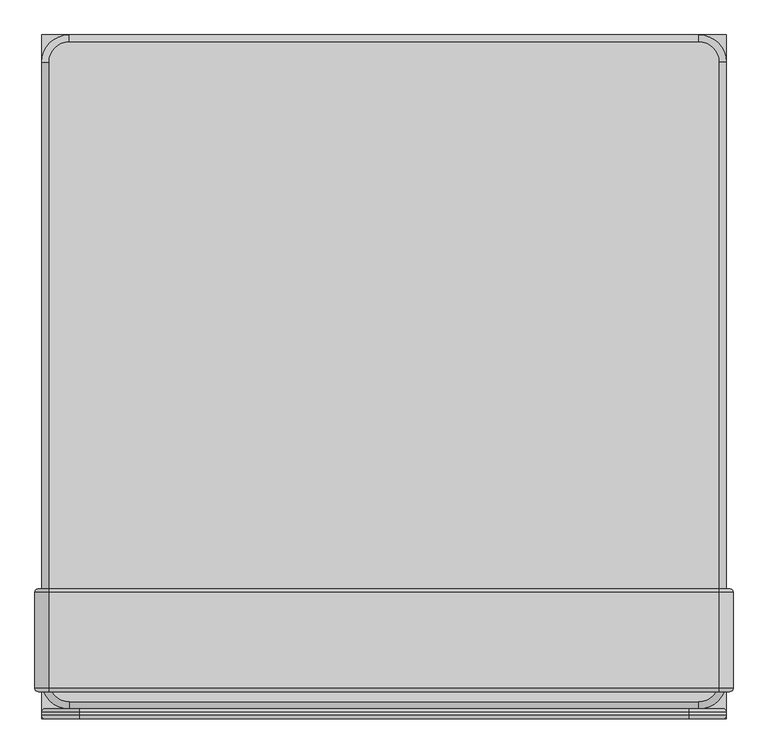
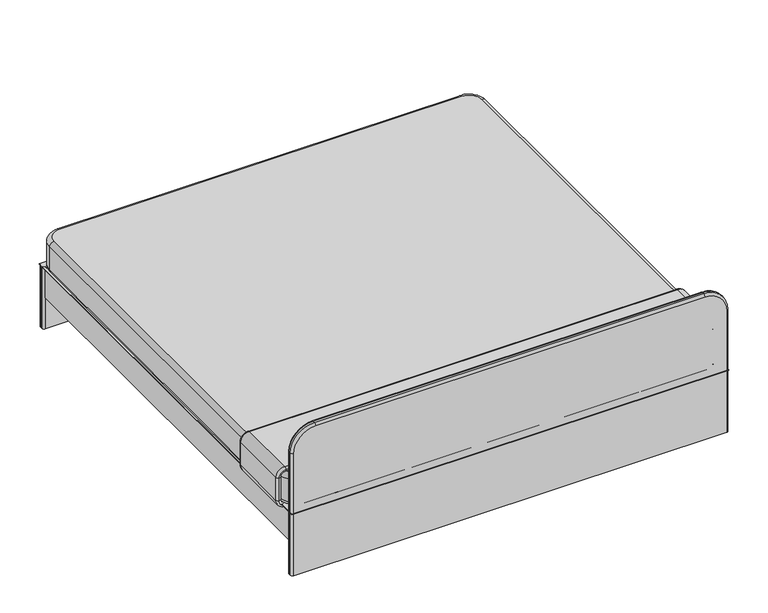
"""IFC4 building model written with IfcOpenShell, lengths in millimetres: furniture geometry, ベッド : 2000 x 2000 mm キング."""

from ifc_helpers import new_model, si_unit, point, frame, frame_2d, origin, origin_with_axes, place, context, project, spatial, polyline, circle_curve, ellipse_curve, trimmed, segment, composite_curve, outline, extrude, source, transform, mapped, element, save
from ifc_brep_helpers import plane_surface, cylinder_surface, revolved_surface, advanced_brep


def furniture_2da6a2a7(model_context):
    return source(origin(), model_context, "Body", "SolidModel", [
        advanced_brep(
        [(1000.0, -960.0, 430.0), (980.0, -960.0, 450.0), (980.0, -680.0, 450.0), (1000.0, -680.0, 430.0), (1010.0, -970.0, 430.0), (980.0, -970.0, 460.0), (1020.0, -960.0, 430.0), (980.0, -960.0, 470.0), (1020.0, -680.0, 430.0), (980.0, -680.0, 470.0), (1010.0, -670.0, 430.0), (980.0, -670.0, 460.0), (1000.0, -680.0, 320.0), (1000.0, -960.0, 320.0), (1010.0, -970.0, 320.0), (1020.0, -960.0, 320.0), (1020.0, -680.0, 320.0), (1010.0, -670.0, 320.0), (980.0, -960.0, 300.0), (980.0, -680.0, 300.0), (980.0, -970.0, 290.0), (980.0, -960.0, 280.0), (980.0, -680.0, 280.0), (980.0, -670.0, 290.0), (-980.0, -680.0, 300.0), (-980.0, -960.0, 300.0), (-980.0, -970.0, 290.0), (-980.0, -960.0, 280.0), (-980.0, -680.0, 280.0), (-980.0, -670.0, 290.0), (-1000.0, -960.0, 320.0), (-1000.0, -680.0, 320.0), (-1010.0, -970.0, 320.0), (-1020.0, -960.0, 320.0), (-1020.0, -680.0, 320.0), (-1010.0, -670.0, 320.0), (-1000.0, -680.0, 430.0), (-1000.0, -960.0, 430.0), (-1010.0, -970.0, 430.0), (-1020.0, -960.0, 430.0), (-1020.0, -680.0, 430.0), (-1010.0, -670.0, 430.0), (-980.0, -960.0, 450.0), (-980.0, -680.0, 450.0), (-980.0, -970.0, 460.0), (-980.0, -960.0, 470.0), (-980.0, -680.0, 470.0), (-980.0, -670.0, 460.0)],
        [
            (0, 1, circle_curve(frame((980.0, -960.0, 430.0), z_axis=(0.0, -1.0, 0.0), x_axis=(0.0, 0.0, 1.0)), 20.0)),
            (1, 2),
            (2, 3, circle_curve(frame((980.0, -680.0, 430.0), z_axis=(0.0, 1.0, 0.0), x_axis=(0.0, 0.0, 1.0)), 20.0)),
            (3, 0),
            (4, 5, circle_curve(frame((980.0, -970.0, 430.0), z_axis=(0.0, -1.0, 0.0), x_axis=(0.0, 0.0, 1.0)), 30.0)),
            (5, 1, circle_curve(frame((980.0, -960.0, 460.0), z_axis=(1.0, 0.0, 0.0), x_axis=(0.0, 0.0, 1.0)), 10.0)),
            (0, 4, circle_curve(frame((1010.0, -960.0, 430.0), z_axis=(0.0, 0.0, 1.0), x_axis=(1.0, 0.0, 0.0)), 10.0)),
            (6, 7, circle_curve(frame((980.0, -960.0, 430.0), z_axis=(0.0, -1.0, 0.0), x_axis=(0.0, 0.0, 1.0)), 40.0)),
            (7, 5, circle_curve(frame((980.0, -960.0, 460.0), z_axis=(1.0, 0.0, 0.0), x_axis=(0.0, 0.0, 1.0)), 10.0)),
            (4, 6, circle_curve(frame((1010.0, -960.0, 430.0), z_axis=(0.0, 0.0, 1.0), x_axis=(1.0, 0.0, 0.0)), 10.0)),
            (8, 9, circle_curve(frame((980.0, -680.0, 430.0), z_axis=(0.0, -1.0, 0.0), x_axis=(0.0, 0.0, 1.0)), 40.0)),
            (9, 7),
            (6, 8),
            (10, 11, circle_curve(frame((980.0, -670.0, 430.0), z_axis=(0.0, -1.0, 0.0), x_axis=(0.0, 0.0, 1.0)), 30.0)),
            (11, 9, circle_curve(frame((980.0, -680.0, 460.0), z_axis=(1.0, 0.0, 0.0), x_axis=(0.0, 0.0, 1.0)), 10.0)),
            (8, 10, circle_curve(frame((1010.0, -680.0, 430.0), z_axis=(0.0, 0.0, 1.0), x_axis=(1.0, 0.0, 0.0)), 10.0)),
            (2, 11, circle_curve(frame((980.0, -680.0, 460.0), z_axis=(1.0, 0.0, 0.0), x_axis=(0.0, 0.0, 1.0)), 10.0)),
            (10, 3, circle_curve(frame((1010.0, -680.0, 430.0), z_axis=(0.0, 0.0, 1.0), x_axis=(1.0, 0.0, 0.0)), 10.0)),
            (3, 12),
            (12, 13),
            (13, 0),
            (13, 14, circle_curve(frame((1010.0, -960.0, 320.0), z_axis=(0.0, 0.0, 1.0), x_axis=(1.0, 0.0, 0.0)), 10.0)),
            (14, 4),
            (14, 15, circle_curve(frame((1010.0, -960.0, 320.0), z_axis=(0.0, 0.0, 1.0), x_axis=(1.0, 0.0, 0.0)), 10.0)),
            (15, 6),
            (15, 16),
            (16, 8),
            (16, 17, circle_curve(frame((1010.0, -680.0, 320.0), z_axis=(0.0, 0.0, 1.0), x_axis=(1.0, 0.0, 0.0)), 10.0)),
            (17, 10),
            (17, 12, circle_curve(frame((1010.0, -680.0, 320.0), z_axis=(0.0, 0.0, 1.0), x_axis=(1.0, 0.0, 0.0)), 10.0)),
            (18, 13, circle_curve(frame((980.0, -960.0, 320.0), z_axis=(0.0, -1.0, 0.0), x_axis=(1.0, 0.0, 0.0)), 20.0)),
            (12, 19, circle_curve(frame((980.0, -680.0, 320.0), z_axis=(0.0, 1.0, 0.0), x_axis=(1.0, 0.0, 0.0)), 20.0)),
            (19, 18),
            (20, 14, circle_curve(frame((980.0, -970.0, 320.0), z_axis=(0.0, -1.0, 0.0), x_axis=(1.0, 0.0, 0.0)), 30.0)),
            (18, 20, circle_curve(frame((980.0, -960.0, 290.0), z_axis=(1.0, 0.0, 0.0), x_axis=(0.0, 0.0, -1.0)), 10.0)),
            (21, 15, circle_curve(frame((980.0, -960.0, 320.0), z_axis=(0.0, -1.0, 0.0), x_axis=(1.0, 0.0, 0.0)), 40.0)),
            (20, 21, circle_curve(frame((980.0, -960.0, 290.0), z_axis=(1.0, 0.0, 0.0), x_axis=(0.0, 0.0, -1.0)), 10.0)),
            (22, 16, circle_curve(frame((980.0, -680.0, 320.0), z_axis=(0.0, -1.0, 0.0), x_axis=(1.0, 0.0, 0.0)), 40.0)),
            (21, 22),
            (23, 17, circle_curve(frame((980.0, -670.0, 320.0), z_axis=(0.0, -1.0, 0.0), x_axis=(1.0, 0.0, 0.0)), 30.0)),
            (22, 23, circle_curve(frame((980.0, -680.0, 290.0), z_axis=(1.0, 0.0, 0.0), x_axis=(0.0, 0.0, -1.0)), 10.0)),
            (23, 19, circle_curve(frame((980.0, -680.0, 290.0), z_axis=(1.0, 0.0, 0.0), x_axis=(0.0, 0.0, -1.0)), 10.0)),
            (19, 24),
            (24, 25),
            (25, 18),
            (25, 26, circle_curve(frame((-980.0, -960.0, 290.0), z_axis=(1.0, 0.0, 0.0), x_axis=(0.0, 0.0, -1.0)), 10.0)),
            (26, 20),
            (26, 27, circle_curve(frame((-980.0, -960.0, 290.0), z_axis=(1.0, 0.0, 0.0), x_axis=(0.0, 0.0, -1.0)), 10.0)),
            (27, 21),
            (27, 28),
            (28, 22),
            (28, 29, circle_curve(frame((-980.0, -680.0, 290.0), z_axis=(1.0, 0.0, 0.0), x_axis=(0.0, 0.0, -1.0)), 10.0)),
            (29, 23),
            (29, 24, circle_curve(frame((-980.0, -680.0, 290.0), z_axis=(1.0, 0.0, 0.0), x_axis=(0.0, 0.0, -1.0)), 10.0)),
            (30, 25, circle_curve(frame((-980.0, -960.0, 320.0), z_axis=(0.0, -1.0, 0.0), x_axis=(0.0, 0.0, -1.0)), 20.0)),
            (24, 31, circle_curve(frame((-980.0, -680.0, 320.0), z_axis=(0.0, 1.0, 0.0), x_axis=(0.0, 0.0, -1.0)), 20.0)),
            (31, 30),
            (32, 26, circle_curve(frame((-980.0, -970.0, 320.0), z_axis=(0.0, -1.0, 0.0), x_axis=(0.0, 0.0, -1.0)), 30.0)),
            (30, 32, circle_curve(frame((-1010.0, -960.0, 320.0), z_axis=(0.0, 0.0, -1.0), x_axis=(-1.0, 0.0, 0.0)), 10.0)),
            (33, 27, circle_curve(frame((-980.0, -960.0, 320.0), z_axis=(0.0, -1.0, 0.0), x_axis=(0.0, 0.0, -1.0)), 40.0)),
            (32, 33, circle_curve(frame((-1010.0, -960.0, 320.0), z_axis=(0.0, 0.0, -1.0), x_axis=(-1.0, 0.0, 0.0)), 10.0)),
            (34, 28, circle_curve(frame((-980.0, -680.0, 320.0), z_axis=(0.0, -1.0, 0.0), x_axis=(0.0, 0.0, -1.0)), 40.0)),
            (33, 34),
            (35, 29, circle_curve(frame((-980.0, -670.0, 320.0), z_axis=(0.0, -1.0, 0.0), x_axis=(0.0, 0.0, -1.0)), 30.0)),
            (34, 35, circle_curve(frame((-1010.0, -680.0, 320.0), z_axis=(0.0, 0.0, -1.0), x_axis=(-1.0, 0.0, 0.0)), 10.0)),
            (35, 31, circle_curve(frame((-1010.0, -680.0, 320.0), z_axis=(0.0, 0.0, -1.0), x_axis=(-1.0, 0.0, 0.0)), 10.0)),
            (31, 36),
            (36, 37),
            (37, 30),
            (37, 38, circle_curve(frame((-1010.0, -960.0, 430.0), z_axis=(0.0, 0.0, -1.0), x_axis=(-1.0, 0.0, 0.0)), 10.0)),
            (38, 32),
            (38, 39, circle_curve(frame((-1010.0, -960.0, 430.0), z_axis=(0.0, 0.0, -1.0), x_axis=(-1.0, 0.0, 0.0)), 10.0)),
            (39, 33),
            (39, 40),
            (40, 34),
            (40, 41, circle_curve(frame((-1010.0, -680.0, 430.0), z_axis=(0.0, 0.0, -1.0), x_axis=(-1.0, 0.0, 0.0)), 10.0)),
            (41, 35),
            (41, 36, circle_curve(frame((-1010.0, -680.0, 430.0), z_axis=(0.0, 0.0, -1.0), x_axis=(-1.0, 0.0, 0.0)), 10.0)),
            (42, 37, circle_curve(frame((-980.0, -960.0, 430.0), z_axis=(0.0, -1.0, 0.0), x_axis=(-1.0, 0.0, 0.0)), 20.0)),
            (36, 43, circle_curve(frame((-980.0, -680.0, 430.0), z_axis=(0.0, 1.0, 0.0), x_axis=(-1.0, 0.0, 0.0)), 20.0)),
            (43, 42),
            (44, 38, circle_curve(frame((-980.0, -970.0, 430.0), z_axis=(0.0, -1.0, 0.0), x_axis=(-1.0, 0.0, 0.0)), 30.0)),
            (42, 44, circle_curve(frame((-980.0, -960.0, 460.0), z_axis=(-1.0, 0.0, 0.0), x_axis=(0.0, 0.0, 1.0)), 10.0)),
            (45, 39, circle_curve(frame((-980.0, -960.0, 430.0), z_axis=(0.0, -1.0, 0.0), x_axis=(-1.0, 0.0, 0.0)), 40.0)),
            (44, 45, circle_curve(frame((-980.0, -960.0, 460.0), z_axis=(-1.0, 0.0, 0.0), x_axis=(0.0, 0.0, 1.0)), 10.0)),
            (46, 40, circle_curve(frame((-980.0, -680.0, 430.0), z_axis=(0.0, -1.0, 0.0), x_axis=(-1.0, 0.0, 0.0)), 40.0)),
            (45, 46),
            (47, 41, circle_curve(frame((-980.0, -670.0, 430.0), z_axis=(0.0, -1.0, 0.0), x_axis=(-1.0, 0.0, 0.0)), 30.0)),
            (46, 47, circle_curve(frame((-980.0, -680.0, 460.0), z_axis=(-1.0, 0.0, 0.0), x_axis=(0.0, 0.0, 1.0)), 10.0)),
            (47, 43, circle_curve(frame((-980.0, -680.0, 460.0), z_axis=(-1.0, 0.0, 0.0), x_axis=(0.0, 0.0, 1.0)), 10.0)),
            (43, 2),
            (1, 42),
            (5, 44),
            (7, 45),
            (9, 46),
            (11, 47),
        ],
        [
            revolved_surface(polyline([(980.0, -680.0, 450.0), (980.0, -960.0, 450.0)]), (980.0, -970.0, 430.0), (0.0, 1.0, 0.0)),
            revolved_surface(trimmed(ellipse_curve(frame((980.0, -960.0, 460.0), z_axis=(-1.0, 0.0, 0.0), x_axis=(0.0, 0.0, 1.0)), 10.0, 10.0), [point((980.0, -960.0, 450.0))], [point((980.0, -970.0, 460.0))], True, "CARTESIAN"), (980.0, -970.0, 430.0), (0.0, 1.0, 0.0)),
            revolved_surface(trimmed(ellipse_curve(frame((980.0, -960.0, 460.0), z_axis=(-1.0, 0.0, 0.0), x_axis=(0.0, 0.0, 1.0)), 10.0, 10.0), [point((980.0, -970.0, 460.0))], [point((980.0, -960.0, 470.0))], True, "CARTESIAN"), (980.0, -970.0, 430.0), (0.0, 1.0, 0.0)),
            cylinder_surface(frame((980.0, -970.0, 430.0), z_axis=(0.0, 1.0, 0.0), x_axis=(0.0, 0.0, 1.0)), 40.0),
            revolved_surface(trimmed(ellipse_curve(frame((980.0, -680.0, 460.0), z_axis=(-1.0, 0.0, 0.0), x_axis=(0.0, 0.0, 1.0)), 10.0, 10.0), [point((980.0, -680.0, 470.0))], [point((980.0, -670.0, 460.0))], True, "CARTESIAN"), (980.0, -970.0, 430.0), (0.0, 1.0, 0.0)),
            revolved_surface(trimmed(ellipse_curve(frame((980.0, -680.0, 460.0), z_axis=(-1.0, 0.0, 0.0), x_axis=(0.0, 0.0, 1.0)), 10.0, 10.0), [point((980.0, -670.0, 460.0))], [point((980.0, -680.0, 450.0))], True, "CARTESIAN"), (980.0, -970.0, 430.0), (0.0, 1.0, 0.0)),
            plane_surface(frame((1000.0, -680.0, 430.0), z_axis=(-1.0, 0.0, 0.0), x_axis=(0.0, 0.0, -1.0))),
            cylinder_surface(frame((1010.0, -960.0, 430.0), z_axis=(0.0, 0.0, 1.0), x_axis=(1.0, 0.0, 0.0)), 10.0),
            plane_surface(frame((1020.0, -960.0, 430.0), z_axis=(1.0, 0.0, 0.0), x_axis=(0.0, 0.0, -1.0))),
            cylinder_surface(frame((1010.0, -680.0, 430.0), z_axis=(0.0, 0.0, 1.0), x_axis=(1.0, 0.0, 0.0)), 10.0),
            revolved_surface(polyline([(1000.0, -680.0, 320.0), (1000.0, -960.0, 320.0)]), (980.0, -970.0, 320.0), (0.0, 1.0, 0.0)),
            revolved_surface(trimmed(ellipse_curve(frame((1010.0, -960.0, 320.0), z_axis=(0.0, 0.0, 1.0), x_axis=(1.0, 0.0, 0.0)), 10.0, 10.0), [point((1000.0, -960.0, 320.0))], [point((1010.0, -970.0, 320.0))], True, "CARTESIAN"), (980.0, -970.0, 320.0), (0.0, 1.0, 0.0)),
            revolved_surface(trimmed(ellipse_curve(frame((1010.0, -960.0, 320.0), z_axis=(0.0, 0.0, 1.0), x_axis=(1.0, 0.0, 0.0)), 10.0, 10.0), [point((1010.0, -970.0, 320.0))], [point((1020.0, -960.0, 320.0))], True, "CARTESIAN"), (980.0, -970.0, 320.0), (0.0, 1.0, 0.0)),
            cylinder_surface(frame((980.0, -970.0, 320.0), z_axis=(0.0, 1.0, 0.0), x_axis=(1.0, 0.0, 0.0)), 40.0),
            revolved_surface(trimmed(ellipse_curve(frame((1010.0, -680.0, 320.0), z_axis=(0.0, 0.0, 1.0), x_axis=(1.0, 0.0, 0.0)), 10.0, 10.0), [point((1020.0, -680.0, 320.0))], [point((1010.0, -670.0, 320.0))], True, "CARTESIAN"), (980.0, -970.0, 320.0), (0.0, 1.0, 0.0)),
            revolved_surface(trimmed(ellipse_curve(frame((1010.0, -680.0, 320.0), z_axis=(0.0, 0.0, 1.0), x_axis=(1.0, 0.0, 0.0)), 10.0, 10.0), [point((1010.0, -670.0, 320.0))], [point((1000.0, -680.0, 320.0))], True, "CARTESIAN"), (980.0, -970.0, 320.0), (0.0, 1.0, 0.0)),
            plane_surface(frame((980.0, -680.0, 300.0), z_axis=(0.0, 0.0, 1.0), x_axis=(-1.0, 0.0, 0.0))),
            cylinder_surface(frame((980.0, -960.0, 290.0), z_axis=(1.0, 0.0, 0.0), x_axis=(0.0, 0.0, -1.0)), 10.0),
            plane_surface(frame((980.0, -960.0, 280.0), z_axis=(0.0, 0.0, -1.0), x_axis=(-1.0, 0.0, 0.0))),
            cylinder_surface(frame((980.0, -680.0, 290.0), z_axis=(1.0, 0.0, 0.0), x_axis=(0.0, 0.0, -1.0)), 10.0),
            revolved_surface(polyline([(-980.0, -680.0, 300.0), (-980.0, -960.0, 300.0)]), (-980.0, -970.0, 320.0), (0.0, 1.0, 0.0)),
            revolved_surface(trimmed(ellipse_curve(frame((-980.0, -960.0, 290.0), z_axis=(1.0, 0.0, 0.0), x_axis=(0.0, 0.0, -1.0)), 10.0, 10.0), [point((-980.0, -960.0, 300.0))], [point((-980.0, -970.0, 290.0))], True, "CARTESIAN"), (-980.0, -970.0, 320.0), (0.0, 1.0, 0.0)),
            revolved_surface(trimmed(ellipse_curve(frame((-980.0, -960.0, 290.0), z_axis=(1.0, 0.0, 0.0), x_axis=(0.0, 0.0, -1.0)), 10.0, 10.0), [point((-980.0, -970.0, 290.0))], [point((-980.0, -960.0, 280.0))], True, "CARTESIAN"), (-980.0, -970.0, 320.0), (0.0, 1.0, 0.0)),
            cylinder_surface(frame((-980.0, -970.0, 320.0), z_axis=(0.0, 1.0, 0.0), x_axis=(0.0, 0.0, -1.0)), 40.0),
            revolved_surface(trimmed(ellipse_curve(frame((-980.0, -680.0, 290.0), z_axis=(1.0, 0.0, 0.0), x_axis=(0.0, 0.0, -1.0)), 10.0, 10.0), [point((-980.0, -680.0, 280.0))], [point((-980.0, -670.0, 290.0))], True, "CARTESIAN"), (-980.0, -970.0, 320.0), (0.0, 1.0, 0.0)),
            revolved_surface(trimmed(ellipse_curve(frame((-980.0, -680.0, 290.0), z_axis=(1.0, 0.0, 0.0), x_axis=(0.0, 0.0, -1.0)), 10.0, 10.0), [point((-980.0, -670.0, 290.0))], [point((-980.0, -680.0, 300.0))], True, "CARTESIAN"), (-980.0, -970.0, 320.0), (0.0, 1.0, 0.0)),
            plane_surface(frame((-1000.0, -680.0, 320.0), z_axis=(1.0, 0.0, 0.0), x_axis=(0.0, 0.0, 1.0))),
            cylinder_surface(frame((-1010.0, -960.0, 320.0), z_axis=(0.0, 0.0, -1.0), x_axis=(-1.0, 0.0, 0.0)), 10.0),
            plane_surface(frame((-1020.0, -960.0, 320.0), z_axis=(-1.0, 0.0, 0.0), x_axis=(0.0, 0.0, 1.0))),
            cylinder_surface(frame((-1010.0, -680.0, 320.0), z_axis=(0.0, 0.0, -1.0), x_axis=(-1.0, 0.0, 0.0)), 10.0),
            revolved_surface(polyline([(-1000.0, -680.0, 430.0), (-1000.0, -960.0, 430.0)]), (-980.0, -970.0, 430.0), (0.0, 1.0, 0.0)),
            revolved_surface(trimmed(ellipse_curve(frame((-1010.0, -960.0, 430.0), z_axis=(0.0, 0.0, -1.0), x_axis=(-1.0, 0.0, 0.0)), 10.0, 10.0), [point((-1000.0, -960.0, 430.0))], [point((-1010.0, -970.0, 430.0))], True, "CARTESIAN"), (-980.0, -970.0, 430.0), (0.0, 1.0, 0.0)),
            revolved_surface(trimmed(ellipse_curve(frame((-1010.0, -960.0, 430.0), z_axis=(0.0, 0.0, -1.0), x_axis=(-1.0, 0.0, 0.0)), 10.0, 10.0), [point((-1010.0, -970.0, 430.0))], [point((-1020.0, -960.0, 430.0))], True, "CARTESIAN"), (-980.0, -970.0, 430.0), (0.0, 1.0, 0.0)),
            cylinder_surface(frame((-980.0, -970.0, 430.0), z_axis=(0.0, 1.0, 0.0), x_axis=(-1.0, 0.0, 0.0)), 40.0),
            revolved_surface(trimmed(ellipse_curve(frame((-1010.0, -680.0, 430.0), z_axis=(0.0, 0.0, -1.0), x_axis=(-1.0, 0.0, 0.0)), 10.0, 10.0), [point((-1020.0, -680.0, 430.0))], [point((-1010.0, -670.0, 430.0))], True, "CARTESIAN"), (-980.0, -970.0, 430.0), (0.0, 1.0, 0.0)),
            revolved_surface(trimmed(ellipse_curve(frame((-1010.0, -680.0, 430.0), z_axis=(0.0, 0.0, -1.0), x_axis=(-1.0, 0.0, 0.0)), 10.0, 10.0), [point((-1010.0, -670.0, 430.0))], [point((-1000.0, -680.0, 430.0))], True, "CARTESIAN"), (-980.0, -970.0, 430.0), (0.0, 1.0, 0.0)),
            plane_surface(frame((-980.0, -680.0, 450.0), z_axis=(0.0, 0.0, -1.0), x_axis=(1.0, 0.0, 0.0))),
            cylinder_surface(frame((-980.0, -960.0, 460.0), z_axis=(-1.0, 0.0, 0.0), x_axis=(0.0, 0.0, 1.0)), 10.0),
            plane_surface(frame((-980.0, -960.0, 470.0), z_axis=(0.0, 0.0, 1.0), x_axis=(1.0, 0.0, 0.0))),
            cylinder_surface(frame((-980.0, -680.0, 460.0), z_axis=(-1.0, 0.0, 0.0), x_axis=(0.0, 0.0, 1.0)), 10.0),
        ],
        [
            (0, [[1, 2, 3, 4]]),
            (1, [[5, 6, -1, 7]]),
            (2, [[8, 9, -5, 10]]),
            (3, [[11, 12, -8, 13]]),
            (4, [[14, 15, -11, 16]]),
            (5, [[-3, 17, -14, 18]]),
            (6, [[-4, 19, 20, 21]]),
            (7, [[-7, -21, 22, 23]]),
            (7, [[-10, -23, 24, 25]]),
            (8, [[-13, -25, 26, 27]]),
            (9, [[-16, -27, 28, 29]]),
            (9, [[-18, -29, 30, -19]]),
            (10, [[31, -20, 32, 33]]),
            (11, [[34, -22, -31, 35]]),
            (12, [[36, -24, -34, 37]]),
            (13, [[38, -26, -36, 39]]),
            (14, [[40, -28, -38, 41]]),
            (15, [[-32, -30, -40, 42]]),
            (16, [[-33, 43, 44, 45]]),
            (17, [[-35, -45, 46, 47]]),
            (17, [[-37, -47, 48, 49]]),
            (18, [[-39, -49, 50, 51]]),
            (19, [[-41, -51, 52, 53]]),
            (19, [[-42, -53, 54, -43]]),
            (20, [[55, -44, 56, 57]]),
            (21, [[58, -46, -55, 59]]),
            (22, [[60, -48, -58, 61]]),
            (23, [[62, -50, -60, 63]]),
            (24, [[64, -52, -62, 65]]),
            (25, [[-56, -54, -64, 66]]),
            (26, [[-57, 67, 68, 69]]),
            (27, [[-59, -69, 70, 71]]),
            (27, [[-61, -71, 72, 73]]),
            (28, [[-63, -73, 74, 75]]),
            (29, [[-65, -75, 76, 77]]),
            (29, [[-66, -77, 78, -67]]),
            (30, [[79, -68, 80, 81]]),
            (31, [[82, -70, -79, 83]]),
            (32, [[84, -72, -82, 85]]),
            (33, [[86, -74, -84, 87]]),
            (34, [[88, -76, -86, 89]]),
            (35, [[-80, -78, -88, 90]]),
            (36, [[-81, 91, -2, 92]]),
            (37, [[-83, -92, -6, 93]]),
            (37, [[-85, -93, -9, 94]]),
            (38, [[-87, -94, -12, 95]]),
            (39, [[-89, -95, -15, 96]]),
            (39, [[-90, -96, -17, -91]]),
        ],
    ),
        extrude(outline(polyline([(1000.0, -1050.0), (-1000.0, -1050.0), (-1000.0, 950.0), (1000.0, 950.0), (1000.0, -1050.0)])), frame((0.0, 0.0, 298.0), z_axis=(0.0, 0.0, 1.0), x_axis=(1.0, 0.0, 0.0)), (0.0, 0.0, 1.0), 2.0),
        advanced_brep(
        [(1000.0, -940.0, 320.0), (920.0, -1020.0, 320.0), (920.0, -1000.0, 300.0), (980.0, -940.0, 300.0), (1000.0, -940.0, 430.0), (920.0, -1020.0, 430.0), (980.0, -940.0, 450.0), (920.0, -1000.0, 450.0), (980.0, 870.0, 300.0), (1000.0, 870.0, 320.0), (1000.0, 870.0, 430.0), (980.0, 870.0, 450.0), (920.0, 930.0, 300.0), (920.0, 950.0, 320.0), (920.0, 950.0, 430.0), (920.0, 930.0, 450.0), (-920.0, 930.0, 300.0), (-920.0, 950.0, 320.0), (-920.0, 950.0, 430.0), (-920.0, 930.0, 450.0), (-980.0, 870.0, 300.0), (-1000.0, 870.0, 320.0), (-1000.0, 870.0, 430.0), (-980.0, 870.0, 450.0), (-980.0, -940.0, 300.0), (-1000.0, -940.0, 320.0), (-1000.0, -940.0, 430.0), (-980.0, -940.0, 450.0), (-920.0, -1000.0, 300.0), (-920.0, -1020.0, 320.0), (-920.0, -1020.0, 430.0), (-920.0, -1000.0, 450.0)],
        [
            (0, 1, circle_curve(frame((920.0, -940.0, 320.0), z_axis=(0.0, 0.0, -1.0), x_axis=(0.0, -1.0, 0.0)), 80.0)),
            (1, 2, circle_curve(frame((920.0, -1000.0, 320.0), z_axis=(1.0, 0.0, 0.0), x_axis=(0.0, 1.0, 0.0)), 20.0)),
            (2, 3, circle_curve(frame((920.0, -940.0, 300.0), z_axis=(0.0, 0.0, 1.0), x_axis=(0.0, -1.0, 0.0)), 60.0)),
            (3, 0, circle_curve(frame((980.0, -940.0, 320.0), z_axis=(0.0, -1.0, 0.0), x_axis=(-1.0, 0.0, 0.0)), 20.0)),
            (0, 4),
            (4, 5, circle_curve(frame((920.0, -940.0, 430.0), z_axis=(0.0, 0.0, -1.0), x_axis=(0.0, -1.0, 0.0)), 80.0)),
            (5, 1),
            (4, 6, circle_curve(frame((980.0, -940.0, 430.0), z_axis=(0.0, -1.0, 0.0), x_axis=(-1.0, 0.0, 0.0)), 20.0)),
            (6, 7, circle_curve(frame((920.0, -940.0, 450.0), z_axis=(0.0, 0.0, -1.0), x_axis=(0.0, -1.0, 0.0)), 60.0)),
            (7, 5, circle_curve(frame((920.0, -1000.0, 430.0), z_axis=(1.0, 0.0, 0.0), x_axis=(0.0, 1.0, 0.0)), 20.0)),
            (3, 8),
            (8, 9, circle_curve(frame((980.0, 870.0, 320.0), z_axis=(0.0, -1.0, 0.0), x_axis=(-1.0, 0.0, 0.0)), 20.0)),
            (9, 0),
            (9, 10),
            (10, 4),
            (10, 11, circle_curve(frame((980.0, 870.0, 430.0), z_axis=(0.0, -1.0, 0.0), x_axis=(-1.0, 0.0, 0.0)), 20.0)),
            (11, 6),
            (8, 12, circle_curve(frame((920.0, 870.0, 300.0), z_axis=(0.0, 0.0, 1.0), x_axis=(1.0, 0.0, 0.0)), 60.0)),
            (12, 13, circle_curve(frame((920.0, 930.0, 320.0), z_axis=(1.0, 0.0, 0.0), x_axis=(0.0, -1.0, 0.0)), 20.0)),
            (13, 9, circle_curve(frame((920.0, 870.0, 320.0), z_axis=(0.0, 0.0, -1.0), x_axis=(1.0, 0.0, 0.0)), 80.0)),
            (13, 14),
            (14, 10, circle_curve(frame((920.0, 870.0, 430.0), z_axis=(0.0, 0.0, -1.0), x_axis=(1.0, 0.0, 0.0)), 80.0)),
            (14, 15, circle_curve(frame((920.0, 930.0, 430.0), z_axis=(1.0, 0.0, 0.0), x_axis=(0.0, -1.0, 0.0)), 20.0)),
            (15, 11, circle_curve(frame((920.0, 870.0, 450.0), z_axis=(0.0, 0.0, -1.0), x_axis=(1.0, 0.0, 0.0)), 60.0)),
            (12, 16),
            (16, 17, circle_curve(frame((-920.0, 930.0, 320.0), z_axis=(1.0, 0.0, 0.0), x_axis=(0.0, -1.0, 0.0)), 20.0)),
            (17, 13),
            (17, 18),
            (18, 14),
            (18, 19, circle_curve(frame((-920.0, 930.0, 430.0), z_axis=(1.0, 0.0, 0.0), x_axis=(0.0, -1.0, 0.0)), 20.0)),
            (19, 15),
            (16, 20, circle_curve(frame((-920.0, 870.0, 300.0), z_axis=(0.0, 0.0, 1.0), x_axis=(0.0, 1.0, 0.0)), 60.0)),
            (20, 21, circle_curve(frame((-980.0, 870.0, 320.0), z_axis=(0.0, 1.0, 0.0), x_axis=(1.0, 0.0, 0.0)), 20.0)),
            (21, 17, circle_curve(frame((-920.0, 870.0, 320.0), z_axis=(0.0, 0.0, -1.0), x_axis=(0.0, 1.0, 0.0)), 80.0)),
            (21, 22),
            (22, 18, circle_curve(frame((-920.0, 870.0, 430.0), z_axis=(0.0, 0.0, -1.0), x_axis=(0.0, 1.0, 0.0)), 80.0)),
            (22, 23, circle_curve(frame((-980.0, 870.0, 430.0), z_axis=(0.0, 1.0, 0.0), x_axis=(1.0, 0.0, 0.0)), 20.0)),
            (23, 19, circle_curve(frame((-920.0, 870.0, 450.0), z_axis=(0.0, 0.0, -1.0), x_axis=(0.0, 1.0, 0.0)), 60.0)),
            (20, 24),
            (24, 25, circle_curve(frame((-980.0, -940.0, 320.0), z_axis=(0.0, 1.0, 0.0), x_axis=(1.0, 0.0, 0.0)), 20.0)),
            (25, 21),
            (25, 26),
            (26, 22),
            (26, 27, circle_curve(frame((-980.0, -940.0, 430.0), z_axis=(0.0, 1.0, 0.0), x_axis=(1.0, 0.0, 0.0)), 20.0)),
            (27, 23),
            (24, 28, circle_curve(frame((-920.0, -940.0, 300.0), z_axis=(0.0, 0.0, 1.0), x_axis=(-1.0, 0.0, 0.0)), 60.0)),
            (28, 29, circle_curve(frame((-920.0, -1000.0, 320.0), z_axis=(-1.0, 0.0, 0.0), x_axis=(0.0, 1.0, 0.0)), 20.0)),
            (29, 25, circle_curve(frame((-920.0, -940.0, 320.0), z_axis=(0.0, 0.0, -1.0), x_axis=(-1.0, 0.0, 0.0)), 80.0)),
            (29, 30),
            (30, 26, circle_curve(frame((-920.0, -940.0, 430.0), z_axis=(0.0, 0.0, -1.0), x_axis=(-1.0, 0.0, 0.0)), 80.0)),
            (30, 31, circle_curve(frame((-920.0, -1000.0, 430.0), z_axis=(-1.0, 0.0, 0.0), x_axis=(0.0, 1.0, 0.0)), 20.0)),
            (31, 27, circle_curve(frame((-920.0, -940.0, 450.0), z_axis=(0.0, 0.0, -1.0), x_axis=(-1.0, 0.0, 0.0)), 60.0)),
            (31, 7),
            (2, 28),
            (1, 29),
            (5, 30),
        ],
        [
            revolved_surface(trimmed(ellipse_curve(frame((920.0, -1000.0, 320.0), z_axis=(-1.0, 0.0, 0.0), x_axis=(0.0, 1.0, 0.0)), 20.0, 20.0), [point((920.0, -1000.0, 300.0))], [point((920.0, -1020.0, 320.0))], True, "CARTESIAN"), (920.0, -940.0, 300.0), (0.0, 0.0, 1.0)),
            cylinder_surface(frame((920.0, -940.0, 300.0), z_axis=(0.0, 0.0, 1.0), x_axis=(0.0, -1.0, 0.0)), 80.0),
            revolved_surface(trimmed(ellipse_curve(frame((920.0, -1000.0, 430.0), z_axis=(-1.0, 0.0, 0.0), x_axis=(0.0, 1.0, 0.0)), 20.0, 20.0), [point((920.0, -1020.0, 430.0))], [point((920.0, -1000.0, 450.0))], True, "CARTESIAN"), (920.0, -940.0, 300.0), (0.0, 0.0, 1.0)),
            cylinder_surface(frame((980.0, -940.0, 320.0), z_axis=(0.0, -1.0, 0.0), x_axis=(-1.0, 0.0, 0.0)), 20.0),
            plane_surface(frame((1000.0, -940.0, 320.0), z_axis=(1.0, 0.0, 0.0), x_axis=(0.0, 1.0, 0.0))),
            cylinder_surface(frame((980.0, -940.0, 430.0), z_axis=(0.0, -1.0, 0.0), x_axis=(-1.0, 0.0, 0.0)), 20.0),
            revolved_surface(trimmed(ellipse_curve(frame((980.0, 870.0, 320.0), z_axis=(0.0, -1.0, 0.0), x_axis=(-1.0, 0.0, 0.0)), 20.0, 20.0), [point((980.0, 870.0, 300.0))], [point((1000.0, 870.0, 320.0))], True, "CARTESIAN"), (920.0, 870.0, 300.0), (0.0, 0.0, 1.0)),
            cylinder_surface(frame((920.0, 870.0, 300.0), z_axis=(0.0, 0.0, 1.0), x_axis=(1.0, 0.0, 0.0)), 80.0),
            revolved_surface(trimmed(ellipse_curve(frame((980.0, 870.0, 430.0), z_axis=(0.0, -1.0, 0.0), x_axis=(-1.0, 0.0, 0.0)), 20.0, 20.0), [point((1000.0, 870.0, 430.0))], [point((980.0, 870.0, 450.0))], True, "CARTESIAN"), (920.0, 870.0, 300.0), (0.0, 0.0, 1.0)),
            cylinder_surface(frame((920.0, 930.0, 320.0), z_axis=(1.0, 0.0, 0.0), x_axis=(0.0, -1.0, 0.0)), 20.0),
            plane_surface(frame((920.0, 950.0, 320.0), z_axis=(0.0, 1.0, 0.0), x_axis=(-1.0, 0.0, 0.0))),
            cylinder_surface(frame((920.0, 930.0, 430.0), z_axis=(1.0, 0.0, 0.0), x_axis=(0.0, -1.0, 0.0)), 20.0),
            revolved_surface(trimmed(ellipse_curve(frame((-920.0, 930.0, 320.0), z_axis=(1.0, 0.0, 0.0), x_axis=(0.0, -1.0, 0.0)), 20.0, 20.0), [point((-920.0, 930.0, 300.0))], [point((-920.0, 950.0, 320.0))], True, "CARTESIAN"), (-920.0, 870.0, 300.0), (0.0, 0.0, 1.0)),
            cylinder_surface(frame((-920.0, 870.0, 300.0), z_axis=(0.0, 0.0, 1.0), x_axis=(0.0, 1.0, 0.0)), 80.0),
            revolved_surface(trimmed(ellipse_curve(frame((-920.0, 930.0, 430.0), z_axis=(1.0, 0.0, 0.0), x_axis=(0.0, -1.0, 0.0)), 20.0, 20.0), [point((-920.0, 950.0, 430.0))], [point((-920.0, 930.0, 450.0))], True, "CARTESIAN"), (-920.0, 870.0, 300.0), (0.0, 0.0, 1.0)),
            cylinder_surface(frame((-980.0, 870.0, 320.0), z_axis=(0.0, 1.0, 0.0), x_axis=(1.0, 0.0, 0.0)), 20.0),
            plane_surface(frame((-1000.0, 870.0, 320.0), z_axis=(-1.0, 0.0, 0.0), x_axis=(0.0, -1.0, 0.0))),
            cylinder_surface(frame((-980.0, 870.0, 430.0), z_axis=(0.0, 1.0, 0.0), x_axis=(1.0, 0.0, 0.0)), 20.0),
            revolved_surface(trimmed(ellipse_curve(frame((-980.0, -940.0, 320.0), z_axis=(0.0, 1.0, 0.0), x_axis=(1.0, 0.0, 0.0)), 20.0, 20.0), [point((-980.0, -940.0, 300.0))], [point((-1000.0, -940.0, 320.0))], True, "CARTESIAN"), (-920.0, -940.0, 300.0), (0.0, 0.0, 1.0)),
            cylinder_surface(frame((-920.0, -940.0, 300.0), z_axis=(0.0, 0.0, 1.0), x_axis=(-1.0, 0.0, 0.0)), 80.0),
            revolved_surface(trimmed(ellipse_curve(frame((-980.0, -940.0, 430.0), z_axis=(0.0, 1.0, 0.0), x_axis=(1.0, 0.0, 0.0)), 20.0, 20.0), [point((-1000.0, -940.0, 430.0))], [point((-980.0, -940.0, 450.0))], True, "CARTESIAN"), (-920.0, -940.0, 300.0), (0.0, 0.0, 1.0)),
            plane_surface(frame((-920.0, -940.0, 450.0), z_axis=(0.0, 0.0, 1.0), x_axis=(-1.0, 0.0, 0.0))),
            plane_surface(frame((-920.0, -940.0, 300.0), z_axis=(0.0, 0.0, -1.0), x_axis=(-1.0, 0.0, 0.0))),
            cylinder_surface(frame((-920.0, -1000.0, 320.0), z_axis=(-1.0, 0.0, 0.0), x_axis=(0.0, 1.0, 0.0)), 20.0),
            plane_surface(frame((-920.0, -1020.0, 320.0), z_axis=(0.0, -1.0, 0.0), x_axis=(1.0, 0.0, 0.0))),
            cylinder_surface(frame((-920.0, -1000.0, 430.0), z_axis=(-1.0, 0.0, 0.0), x_axis=(0.0, 1.0, 0.0)), 20.0),
        ],
        [
            (0, [[1, 2, 3, 4]]),
            (1, [[-1, 5, 6, 7]]),
            (2, [[-6, 8, 9, 10]]),
            (3, [[-4, 11, 12, 13]]),
            (4, [[-5, -13, 14, 15]]),
            (5, [[-8, -15, 16, 17]]),
            (6, [[-12, 18, 19, 20]]),
            (7, [[-14, -20, 21, 22]]),
            (8, [[-16, -22, 23, 24]]),
            (9, [[-19, 25, 26, 27]]),
            (10, [[-21, -27, 28, 29]]),
            (11, [[-23, -29, 30, 31]]),
            (12, [[-26, 32, 33, 34]]),
            (13, [[-28, -34, 35, 36]]),
            (14, [[-30, -36, 37, 38]]),
            (15, [[-33, 39, 40, 41]]),
            (16, [[-35, -41, 42, 43]]),
            (17, [[-37, -43, 44, 45]]),
            (18, [[-40, 46, 47, 48]]),
            (19, [[-42, -48, 49, 50]]),
            (20, [[-44, -50, 51, 52]]),
            (21, [[-9, -17, -24, -31, -38, -45, -52, 53]]),
            (22, [[-3, 54, -46, -39, -32, -25, -18, -11]]),
            (23, [[-2, 55, -47, -54]]),
            (24, [[-7, 56, -49, -55]]),
            (25, [[-10, -53, -51, -56]]),
        ],
    ),
        extrude(outline(polyline([(990.0, -1020.0), (-990.0, -1020.0), (-990.0, 920.0), (990.0, 920.0), (990.0, -1020.0)])), frame((0.0, 0.0, 150.0), z_axis=(0.0, 0.0, 1.0), x_axis=(1.0, 0.0, 0.0)), (0.0, 0.0, 1.0), 150.0),
        extrude(outline(composite_curve([segment(trimmed(circle_curve(frame_2d((990.0, 940.0)), 10.0), [point((990.0, 950.0))], [point((1000.0, 940.0))], False, "CARTESIAN"), True, "CONTINUOUS"), segment(polyline([(1000.0, 940.0), (1000.0, 930.0)]), True, "CONTINUOUS"), segment(trimmed(circle_curve(frame_2d((990.0, 930.0)), 10.0), [point((1000.0, 930.0))], [point((990.0, 920.0))], False, "CARTESIAN"), True, "CONTINUOUS"), segment(polyline([(990.0, 920.0), (-990.0, 920.0)]), True, "CONTINUOUS"), segment(trimmed(circle_curve(frame_2d((-990.0, 930.0)), 10.0), [point((-990.0, 920.0))], [point((-1000.0, 930.0))], False, "CARTESIAN"), True, "CONTINUOUS"), segment(polyline([(-1000.0, 930.0), (-1000.0, 940.0)]), True, "CONTINUOUS"), segment(trimmed(circle_curve(frame_2d((-990.0, 940.0)), 10.0), [point((-1000.0, 940.0))], [point((-990.0, 950.0))], False, "CARTESIAN"), True, "CONTINUOUS"), segment(polyline([(-990.0, 950.0), (990.0, 950.0)]), True, "CONTINUOUS")], self_intersect=False)), origin_with_axes(), (0.0, 0.0, 1.0), 300.0),
        advanced_brep(
        [(-990.0, -1050.0, 0.0), (-1000.0, -1040.0, 0.0), (-1000.0, -1030.0, 0.0), (-990.0, -1020.0, 0.0), (990.0, -1020.0, 0.0), (1000.0, -1030.0, 0.0), (1000.0, -1040.0, 0.0), (990.0, -1050.0, 0.0), (990.0, -1050.0, 590.0), (890.0, -1050.0, 690.0), (-890.0, -1050.0, 690.0), (-990.0, -1050.0, 590.0), (-1000.0, -1040.0, 590.0), (-1000.0, -1030.0, 590.0), (-990.0, -1020.0, 590.0), (-890.0, -1020.0, 690.0), (890.0, -1020.0, 690.0), (990.0, -1020.0, 590.0), (-890.0, -1040.0, 700.0), (-890.0, -1030.0, 700.0), (890.0, -1040.0, 700.0), (890.0, -1030.0, 700.0), (1000.0, -1040.0, 590.0), (1000.0, -1030.0, 590.0)],
        [
            (0, 1, circle_curve(frame((-990.0, -1040.0, 0.0), z_axis=(0.0, 0.0, -1.0), x_axis=(-1.0, 0.0, 0.0)), 10.0)),
            (1, 2),
            (2, 3, circle_curve(frame((-990.0, -1030.0, 0.0), z_axis=(0.0, 0.0, -1.0), x_axis=(-1.0, 0.0, 0.0)), 10.0)),
            (3, 4),
            (4, 5, circle_curve(frame((990.0, -1030.0, 0.0), z_axis=(0.0, 0.0, -1.0), x_axis=(1.0, 0.0, 0.0)), 10.0)),
            (5, 6),
            (6, 7, circle_curve(frame((990.0, -1040.0, 0.0), z_axis=(0.0, 0.0, -1.0), x_axis=(1.0, 0.0, 0.0)), 10.0)),
            (7, 0),
            (7, 8),
            (8, 9, circle_curve(frame((890.0, -1050.0, 590.0), z_axis=(0.0, -1.0, 0.0), x_axis=(0.0, 0.0, 1.0)), 100.0)),
            (9, 10),
            (10, 11, circle_curve(frame((-890.0, -1050.0, 590.0), z_axis=(0.0, -1.0, 0.0), x_axis=(-1.0, 0.0, 0.0)), 100.0)),
            (11, 0),
            (11, 12, circle_curve(frame((-990.0, -1040.0, 590.0), z_axis=(0.0, 0.0, -1.0), x_axis=(-1.0, 0.0, 0.0)), 10.0)),
            (12, 1),
            (12, 13),
            (13, 2),
            (13, 14, circle_curve(frame((-990.0, -1030.0, 590.0), z_axis=(0.0, 0.0, -1.0), x_axis=(-1.0, 0.0, 0.0)), 10.0)),
            (14, 3),
            (14, 15, circle_curve(frame((-890.0, -1020.0, 590.0), z_axis=(0.0, 1.0, 0.0), x_axis=(-1.0, 0.0, 0.0)), 100.0)),
            (15, 16),
            (16, 17, circle_curve(frame((890.0, -1020.0, 590.0), z_axis=(0.0, 1.0, 0.0), x_axis=(0.0, 0.0, 1.0)), 100.0)),
            (17, 4),
            (10, 18, circle_curve(frame((-890.0, -1040.0, 690.0), z_axis=(-1.0, 0.0, 0.0), x_axis=(0.0, 0.0, 1.0)), 10.0)),
            (18, 12, circle_curve(frame((-890.0, -1040.0, 590.0), z_axis=(0.0, -1.0, 0.0), x_axis=(-1.0, 0.0, 0.0)), 110.0)),
            (18, 19),
            (19, 13, circle_curve(frame((-890.0, -1030.0, 590.0), z_axis=(0.0, -1.0, 0.0), x_axis=(-1.0, 0.0, 0.0)), 110.0)),
            (19, 15, circle_curve(frame((-890.0, -1030.0, 690.0), z_axis=(-1.0, 0.0, 0.0), x_axis=(0.0, 0.0, 1.0)), 10.0)),
            (9, 20, circle_curve(frame((890.0, -1040.0, 690.0), z_axis=(-1.0, 0.0, 0.0), x_axis=(0.0, 0.0, 1.0)), 10.0)),
            (20, 18),
            (20, 21),
            (21, 19),
            (21, 16, circle_curve(frame((890.0, -1030.0, 690.0), z_axis=(-1.0, 0.0, 0.0), x_axis=(0.0, 0.0, 1.0)), 10.0)),
            (8, 22, circle_curve(frame((990.0, -1040.0, 590.0), z_axis=(0.0, 0.0, 1.0), x_axis=(1.0, 0.0, 0.0)), 10.0)),
            (22, 20, circle_curve(frame((890.0, -1040.0, 590.0), z_axis=(0.0, -1.0, 0.0), x_axis=(0.0, 0.0, 1.0)), 110.0)),
            (22, 23),
            (23, 21, circle_curve(frame((890.0, -1030.0, 590.0), z_axis=(0.0, -1.0, 0.0), x_axis=(0.0, 0.0, 1.0)), 110.0)),
            (23, 17, circle_curve(frame((990.0, -1030.0, 590.0), z_axis=(0.0, 0.0, 1.0), x_axis=(1.0, 0.0, 0.0)), 10.0)),
            (6, 22),
            (5, 23),
        ],
        [
            plane_surface(frame((-940.0, -1113.2455532, 0.0), z_axis=(0.0, 0.0, -1.0), x_axis=(1.0, 0.0, 0.0))),
            plane_surface(frame((-940.0, -1050.0, 0.0), z_axis=(0.0, -1.0, 0.0), x_axis=(0.0, 0.0, 1.0))),
            cylinder_surface(frame((-990.0, -1040.0, 0.0), z_axis=(0.0, 0.0, -1.0), x_axis=(-1.0, 0.0, 0.0)), 10.0),
            plane_surface(frame((-1000.0, -1040.0, 0.0), z_axis=(-1.0, 0.0, 0.0), x_axis=(0.0, 0.0, 1.0))),
            cylinder_surface(frame((-990.0, -1030.0, 0.0), z_axis=(0.0, 0.0, -1.0), x_axis=(-1.0, 0.0, 0.0)), 10.0),
            plane_surface(frame((-990.0, -1020.0, 0.0), z_axis=(0.0, 1.0, 0.0), x_axis=(0.0, 0.0, 1.0))),
            revolved_surface(trimmed(ellipse_curve(frame((-990.0, -1040.0, 590.0), z_axis=(0.0, 0.0, -1.0), x_axis=(-1.0, 0.0, 0.0)), 10.0, 10.0), [point((-990.0, -1050.0, 590.0))], [point((-1000.0, -1040.0, 590.0))], True, "CARTESIAN"), (-890.0, -1050.0, 590.0), (0.0, 1.0, 0.0)),
            cylinder_surface(frame((-890.0, -1050.0, 590.0), z_axis=(0.0, 1.0, 0.0), x_axis=(-1.0, 0.0, 0.0)), 110.0),
            revolved_surface(trimmed(ellipse_curve(frame((-990.0, -1030.0, 590.0), z_axis=(0.0, 0.0, -1.0), x_axis=(-1.0, 0.0, 0.0)), 10.0, 10.0), [point((-1000.0, -1030.0, 590.0))], [point((-990.0, -1020.0, 590.0))], True, "CARTESIAN"), (-890.0, -1050.0, 590.0), (0.0, 1.0, 0.0)),
            cylinder_surface(frame((-890.0, -1040.0, 690.0), z_axis=(-1.0, 0.0, 0.0), x_axis=(0.0, 0.0, 1.0)), 10.0),
            plane_surface(frame((-890.0, -1040.0, 700.0), z_axis=(0.0, 0.0, 1.0), x_axis=(1.0, 0.0, 0.0))),
            cylinder_surface(frame((-890.0, -1030.0, 690.0), z_axis=(-1.0, 0.0, 0.0), x_axis=(0.0, 0.0, 1.0)), 10.0),
            revolved_surface(trimmed(ellipse_curve(frame((890.0, -1040.0, 690.0), z_axis=(-1.0, 0.0, 0.0), x_axis=(0.0, 0.0, 1.0)), 10.0, 10.0), [point((890.0, -1050.0, 690.0))], [point((890.0, -1040.0, 700.0))], True, "CARTESIAN"), (890.0, -1050.0, 590.0), (0.0, 1.0, 0.0)),
            cylinder_surface(frame((890.0, -1050.0, 590.0), z_axis=(0.0, 1.0, 0.0), x_axis=(0.0, 0.0, 1.0)), 110.0),
            revolved_surface(trimmed(ellipse_curve(frame((890.0, -1030.0, 690.0), z_axis=(-1.0, 0.0, 0.0), x_axis=(0.0, 0.0, 1.0)), 10.0, 10.0), [point((890.0, -1030.0, 700.0))], [point((890.0, -1020.0, 690.0))], True, "CARTESIAN"), (890.0, -1050.0, 590.0), (0.0, 1.0, 0.0)),
            cylinder_surface(frame((990.0, -1040.0, 590.0), z_axis=(0.0, 0.0, 1.0), x_axis=(1.0, 0.0, 0.0)), 10.0),
            plane_surface(frame((1000.0, -1040.0, 590.0), z_axis=(1.0, 0.0, 0.0), x_axis=(0.0, 0.0, -1.0))),
            cylinder_surface(frame((990.0, -1030.0, 590.0), z_axis=(0.0, 0.0, 1.0), x_axis=(1.0, 0.0, 0.0)), 10.0),
        ],
        [
            (0, [[1, 2, 3, 4, 5, 6, 7, 8]]),
            (1, [[-8, 9, 10, 11, 12, 13]]),
            (2, [[-1, -13, 14, 15]]),
            (3, [[-2, -15, 16, 17]]),
            (4, [[-3, -17, 18, 19]]),
            (5, [[-4, -19, 20, 21, 22, 23]]),
            (6, [[-12, 24, 25, -14]]),
            (7, [[-16, -25, 26, 27]]),
            (8, [[-18, -27, 28, -20]]),
            (9, [[-11, 29, 30, -24]]),
            (10, [[-26, -30, 31, 32]]),
            (11, [[-21, -28, -32, 33]]),
            (12, [[-10, 34, 35, -29]]),
            (13, [[-31, -35, 36, 37]]),
            (14, [[-22, -33, -37, 38]]),
            (15, [[-9, -7, 39, -34]]),
            (16, [[-36, -39, -6, 40]]),
            (17, [[-23, -38, -40, -5]]),
        ],
    ),
    ])


if __name__ == "__main__":
    model = new_model("IFC4")
    model_context = context("Model", 3, world=origin())
    ifc_project = project(units=[si_unit("LENGTHUNIT", "METRE", prefix="MILLI")], contexts=[model_context])
    site = spatial("IfcSite", under=ifc_project)
    building = spatial("IfcBuilding", under=site)
    placement = place(None, origin())
    furniture_shape = furniture_2da6a2a7(model_context)
    element("IfcFurniture", 1, ObjectType="ベッド : 2000 x 2000 mm キング", at=placement, inside=building, context=model_context, shape_type="MappedRepresentation", body=[
        mapped(furniture_shape, transform((0.0, 0.0, 0.0), x_axis=(1.0, 0.0, 0.0), y_axis=(0.0, 1.0, 0.0), z_axis=(0.0, 0.0, 1.0))),
    ])
    save(model, "model.ifc")

# Revit data of these elements
# Type "ベッド : 2000 x 2000 mm キング"
#   Keynote = "12490.FF1"
#   幅 = 2000 mm
#   奥行き = 2000 mm
#   本体 = 木目 - ナチュラル
#   シーツ = モチアミ - 無地 - ホワイト
#   Default Elevation = 0
# Element 1 (IfcFurniture, "ベッド : 2000 x 2000 mm キング")
#   Materials on its faces: "モチアミ - 無地 - ホワイト", "木目 - ナチュラル"
# Materials
#   "木目 - ナチュラル": class "木材", colour RGB 204 173 122, transparency 0, Cost = 0
#   "モチアミ - 無地 - ホワイト": class "モチアミ", colour RGB 239 232 223, transparency 0, Cost = 0
